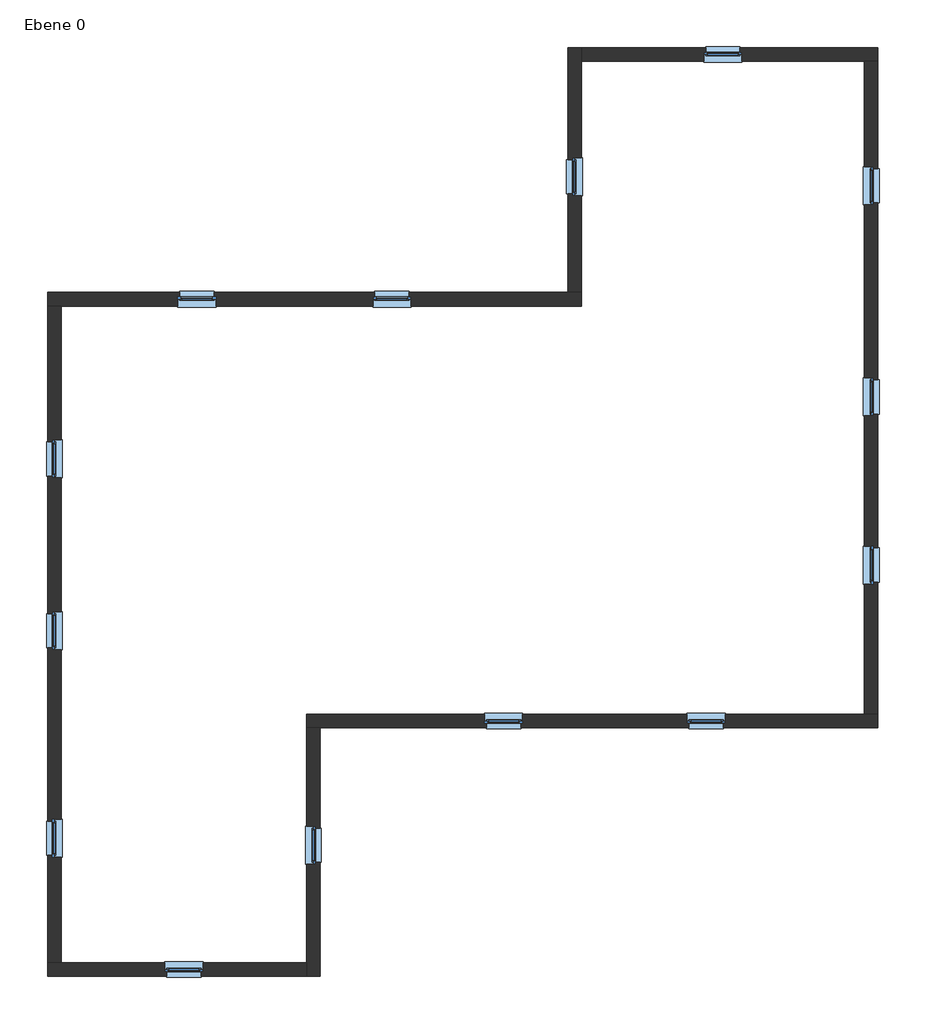
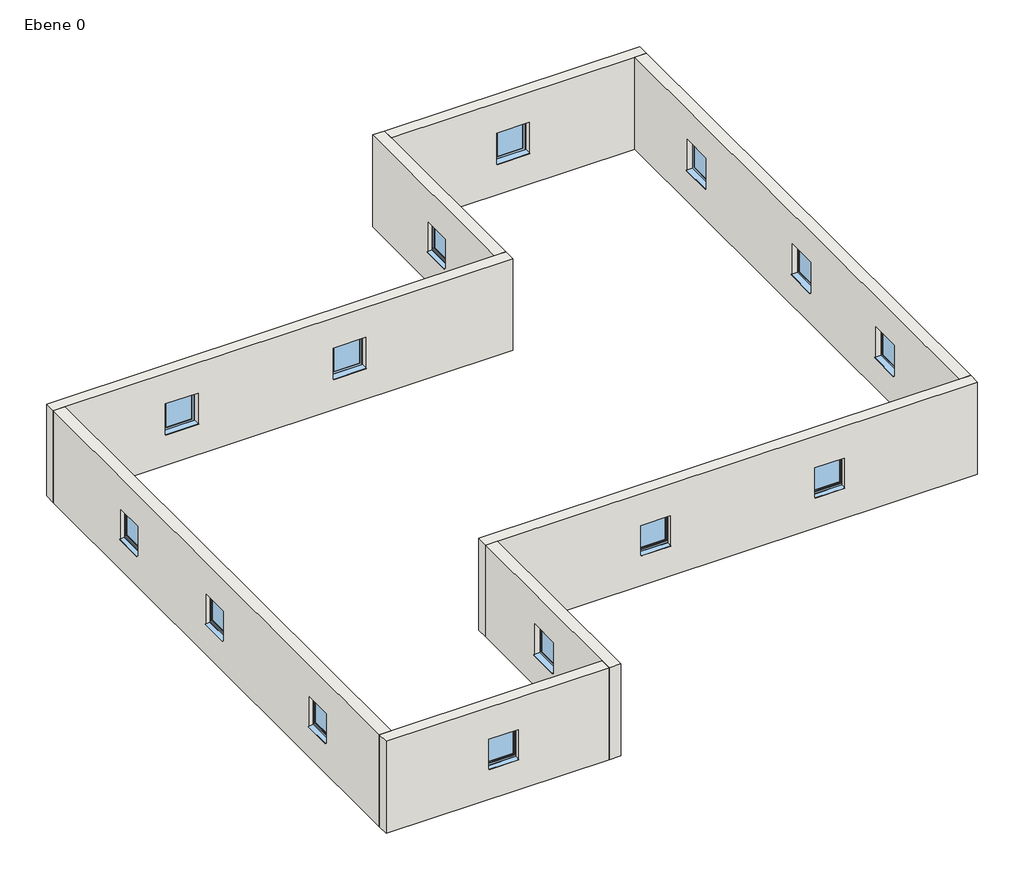
# One storey: 14 windows, 8 walls.
"""IFC4 building model written with IfcOpenShell, lengths in millimetres."""

import ifcopenshell
import ifcopenshell.guid

model = None  # the IFC model being written
_history = None  # IfcOwnerHistory: only IFC2X3 demands one
_inside = {}  # id of a spatial element -> (the spatial element, [elements in it])
_under = {}  # id of a project, library or spatial element -> (it, [spatial elements below it])
_declared = {}  # id of a project -> (the project, [libraries it declares])
_typed = {}  # id of a type object -> (the type object, [elements of that type])
_made_of = {}  # id of a material, layer set ... -> (it, [elements and type objects made of it])


def new_model(schema):
    """Start an empty IFC model of exactly this schema.

    Asked for "IFC4X3", IfcOpenShell would pick the latest addendum, in which some entities
    have other attributes; the version numbers below select the first issue.
    IFC2X3 requires an IfcOwnerHistory on every rooted entity: one is made here for all.
    """
    global model, _history
    if schema == "IFC4X3":
        model = ifcopenshell.file(schema_version=(4, 3, 0, 0))
    else:
        model = ifcopenshell.file(schema=schema)
    _inside.clear()
    _under.clear()
    _declared.clear()
    _typed.clear()
    _made_of.clear()
    _history = None
    if model.schema == "IFC2X3":
        org = make("IfcOrganization", Name="unknown")
        user = make(
            "IfcPersonAndOrganization",
            ThePerson=make("IfcPerson", FamilyName="unknown"),
            TheOrganization=org,
        )
        app = make(
            "IfcApplication",
            ApplicationDeveloper=org,
            Version="unknown",
            ApplicationFullName="unknown",
            ApplicationIdentifier="unknown",
        )
        _history = make(
            "IfcOwnerHistory",
            OwningUser=user,
            OwningApplication=app,
            ChangeAction="ADDED",
            CreationDate=0,
        )
    return model


def make(cls, **values):
    """One entity of the class cls with the attributes given. An attribute that is None is left unset."""
    return model.create_entity(
        cls, **{name: value for name, value in values.items() if value is not None}
    )


def rooted(cls, **values):
    """An entity with a GlobalId (a new one), such as an element, a storey or a relation."""
    return make(cls, GlobalId=ifcopenshell.guid.new(), OwnerHistory=_history, **values)


def si_unit(unit_type, name, prefix=None):
    """IfcSIUnit, for example si_unit("LENGTHUNIT", "METRE", prefix="MILLI")."""
    return make("IfcSIUnit", UnitType=unit_type, Prefix=prefix, Name=name)


def assignment(units):
    """IfcUnitAssignment: the units of a project."""
    return None if units is None else make("IfcUnitAssignment", Units=units)


def point(xyz):
    """IfcCartesianPoint."""
    return None if xyz is None else make("IfcCartesianPoint", Coordinates=xyz)


def direction(xyz):
    """IfcDirection."""
    return None if xyz is None else make("IfcDirection", DirectionRatios=xyz)


def frame(location, z_axis=None, x_axis=None):
    """IfcAxis2Placement3D, a coordinate frame: its origin and axes. An axis left out is left unset."""
    return make(
        "IfcAxis2Placement3D",
        Location=point(location),
        Axis=direction(z_axis),
        RefDirection=direction(x_axis),
    )


def origin():
    """The frame at (0, 0, 0) with its axes left unset."""
    return frame((0.0, 0.0, 0.0))


def place(relative_to, where):
    """IfcLocalPlacement: puts the frame where relative to a parent placement (None: the world)."""
    return make(
        "IfcLocalPlacement", PlacementRelTo=relative_to, RelativePlacement=where
    )


def context(
    kind, dimensions, precision=None, world=None, true_north=None, identifier=None
):
    """IfcGeometricRepresentationContext, for example the 3D "Model" context."""
    return make(
        "IfcGeometricRepresentationContext",
        ContextIdentifier=identifier,
        ContextType=kind,
        CoordinateSpaceDimension=dimensions,
        Precision=precision,
        WorldCoordinateSystem=world,
        TrueNorth=true_north,
    )


def project(units=None, contexts=None):
    """IfcProject with its units and contexts."""
    return rooted(
        "IfcProject",
        Name="project",
        RepresentationContexts=contexts,
        UnitsInContext=assignment(units),
    )


def spatial(cls, under=None, at=None, **own):
    """A site, building, storey or space (cls), placed at a placement, below another one or the project."""
    s = rooted(cls, ObjectPlacement=at, **own)
    if under is not None:
        _under.setdefault(under.id(), (under, []))[1].append(s)
    return s


def polyline(points):
    """IfcPolyline through the points."""
    return make("IfcPolyline", Points=[point(p) for p in points])


def outline(outer, holes=None, kind="AREA"):
    """IfcArbitraryClosedProfileDef: a profile drawn as a closed curve; with holes, ...WithVoids."""
    if holes is None:
        return make("IfcArbitraryClosedProfileDef", ProfileType=kind, OuterCurve=outer)
    return make(
        "IfcArbitraryProfileDefWithVoids",
        ProfileType=kind,
        OuterCurve=outer,
        InnerCurves=holes,
    )


def extrude(swept, where, along, depth):
    """IfcExtrudedAreaSolid: the profile swept, set in the frame where, extruded along a direction by depth."""
    return make(
        "IfcExtrudedAreaSolid",
        SweptArea=swept,
        Position=where,
        ExtrudedDirection=direction(along),
        Depth=depth,
    )


def faces_of(points, faces, orient=None, outer=None):
    """IfcFace entities. A face is a list of loops; a loop is a list of indices into points, from 0.

    orient and outer hold one flag for each loop. By default every Orientation is true, the
    first loop of a face is its IfcFaceOuterBound and the others are IfcFaceBound.
    """
    made = []
    for i, loops in enumerate(faces):
        bounds = []
        for j, loop in enumerate(loops):
            is_outer = j == 0 if outer is None else outer[i][j]
            bounds.append(
                make(
                    "IfcFaceOuterBound" if is_outer else "IfcFaceBound",
                    Bound=make("IfcPolyLoop", Polygon=[points[k] for k in loop]),
                    Orientation=True if orient is None else orient[i][j],
                )
            )
        made.append(make("IfcFace", Bounds=bounds))
    return made


def faceted_brep(points, faces, orient=None, outer=None, voids=None):
    """IfcFacetedBrep: a solid bounded by flat faces; with voids (closed shells), ...WithVoids."""
    shared = [point(p) for p in points]
    hull = make("IfcClosedShell", CfsFaces=faces_of(shared, faces, orient, outer))
    if voids is None:
        return make("IfcFacetedBrep", Outer=hull)
    return make(
        "IfcFacetedBrepWithVoids",
        Outer=hull,
        Voids=[
            make(cls, CfsFaces=faces_of(shared, fs, o, b)) for cls, fs, o, b in voids
        ],
    )


def shape(context_of_items, identifier, shape_type, items):
    """IfcShapeRepresentation: the items that make up one representation, for example the "Body"."""
    return make(
        "IfcShapeRepresentation",
        ContextOfItems=context_of_items,
        RepresentationIdentifier=identifier,
        RepresentationType=shape_type,
        Items=items,
    )


def source(mapping_origin, context_of_items, identifier, shape_type, items):
    """IfcRepresentationMap: a shape defined once, which mapped items show again and again."""
    return make(
        "IfcRepresentationMap",
        MappingOrigin=mapping_origin,
        MappedRepresentation=shape(context_of_items, identifier, shape_type, items),
    )


def transform(
    local_origin,
    x_axis=None,
    y_axis=None,
    z_axis=None,
    scale=None,
    scale2=None,
    scale3=None,
    uniform=True,
):
    """IfcCartesianTransformationOperator3D, or its non-uniform kind. x_axis, y_axis, z_axis: its Axis1, 2, 3."""
    if uniform:
        return make(
            "IfcCartesianTransformationOperator3D",
            Axis1=direction(x_axis),
            Axis2=direction(y_axis),
            LocalOrigin=point(local_origin),
            Scale=scale,
            Axis3=direction(z_axis),
        )
    return make(
        "IfcCartesianTransformationOperator3DnonUniform",
        Axis1=direction(x_axis),
        Axis2=direction(y_axis),
        LocalOrigin=point(local_origin),
        Scale=scale,
        Axis3=direction(z_axis),
        Scale2=scale2,
        Scale3=scale3,
    )


def mapped(mapping_source, mapping_target):
    """IfcMappedItem: shows the shape of a source again, moved by a transform."""
    return make(
        "IfcMappedItem", MappingSource=mapping_source, MappingTarget=mapping_target
    )


def made_of(thing, what):
    """Note that an element or type object is made of a material, layer set ...; save() writes the relation."""
    if what is not None:
        _made_of.setdefault(what.id(), (what, []))[1].append(thing)
    return thing


def element(
    cls,
    number,
    at=None,
    inside=None,
    cuts=None,
    type_object=None,
    material=None,
    context=None,
    identifier="Body",
    shape_type=None,
    held_by="IfcProductDefinitionShape",
    body=None,
    shapes=None,
    **own,
):
    """One element of the class cls, such as IfcWall. Its Tag is "e" and its number.

    at: its placement. inside: the storey or other place that contains it. cuts: it is an
    opening in that element (IfcRelVoidsElement). A single representation is given by context,
    identifier, shape_type and body (its items); several are given by shapes. held_by: the class
    of the entity that holds the representations. save() writes the other relations.
    """
    e = rooted(cls, Tag="e%d" % number, ObjectPlacement=at, **own)
    if body is not None:
        shapes = [shape(context, identifier, shape_type, body)]
    if shapes is not None:
        e.Representation = make(held_by, Representations=shapes)
    if inside is not None:
        _inside.setdefault(inside.id(), (inside, []))[1].append(e)
    if cuts is not None:
        rooted(
            "IfcRelVoidsElement", RelatingBuildingElement=cuts, RelatedOpeningElement=e
        )
    if type_object is not None:
        _typed.setdefault(type_object.id(), (type_object, []))[1].append(e)
    return made_of(e, material)


def aggregate(whole, parts):
    """IfcRelAggregates: a whole, such as a stair, and the parts it consists of."""
    return rooted("IfcRelAggregates", RelatingObject=whole, RelatedObjects=parts)


def save(model, path):
    """Write the relations noted so far, then the file.

    IfcRelAggregates (storeys below a building ...), IfcRelContainedInSpatialStructure (elements
    in a storey), IfcRelDefinesByType, IfcRelAssociatesMaterial and IfcRelDeclares: one each for
    every whole, place, type object, material and project.
    """
    for whole, parts in _under.values():
        aggregate(whole, parts)
    for where, things in _inside.values():
        rooted(
            "IfcRelContainedInSpatialStructure",
            RelatedElements=things,
            RelatingStructure=where,
        )
    for kind, things in _typed.values():
        rooted("IfcRelDefinesByType", RelatedObjects=things, RelatingType=kind)
    for what, things in _made_of.values():
        rooted("IfcRelAssociatesMaterial", RelatedObjects=things, RelatingMaterial=what)
    for by, libraries in _declared.values():
        rooted("IfcRelDeclares", RelatingContext=by, RelatedDefinitions=libraries)
    model.write(path)


def window_1_01_x_1_01_b7243dc8(model_context):
    return source(origin(), model_context, "Body", "SolidModel", [
        extrude(outline(polyline([(-525.0, -210.0), (-525.0, 0.0), (485.0, 0.0), (485.0, -210.0), (-525.0, -210.0)])), frame((0.0, 0.0, 1005.0), z_axis=(0.0, 0.0, 1.0), x_axis=(1.0, 0.0, 0.0)), (0.0, 0.0, 1.0), 15.0),
        extrude(outline(polyline([(375.0, -15.0), (-415.0, -15.0), (-415.0, 15.0), (375.0, 15.0), (375.0, -15.0)])), frame((0.0, 0.0, 1110.0), z_axis=(0.0, 0.0, 1.0), x_axis=(1.0, 0.0, 0.0)), (0.0, 0.0, 1.0), 790.0),
        extrude(outline(polyline([(70.0221543, 1020.0), (210.0, 1000.0), (210.0, 990.0), (208.0, 990.0), (208.0, 998.3604634), (69.8240723, 1018.0), (60.0, 1018.0), (60.0, 1020.0), (70.0221543, 1020.0)])), frame((-475.0, 0.0, 0.0), z_axis=(1.0, 0.0, 0.0), x_axis=(0.0, 1.0, 0.0)), (0.0, 0.0, 1.0), 910.0),
        extrude(outline(polyline([(2010.0, 485.0), (2010.0, -525.0), (1000.0, -525.0), (1000.0, 485.0), (2010.0, 485.0)]), holes=[polyline([(1930.0, 405.0), (1080.0, 405.0), (1080.0, -445.0), (1930.0, -445.0), (1930.0, 405.0)])]), frame((0.0, 0.0, 0.0), z_axis=(0.0, 1.0, 0.0), x_axis=(0.0, 0.0, 1.0)), (0.0, 0.0, 1.0), 60.0),
        faceted_brep([(435.0, 0.0, 1960.0), (435.0, -30.0, 1960.0), (435.0, -30.0, 1050.0), (435.0, 0.0, 1050.0), (-475.0, -30.0, 1960.0), (-475.0, -30.0, 1050.0), (375.0, -30.0, 1110.0), (-415.0, -30.0, 1110.0), (-415.0, -30.0, 1900.0), (375.0, -30.0, 1900.0), (-475.0, 0.0, 1050.0), (-475.0, 0.0, 1960.0), (405.0, 0.0, 1930.0), (-445.0, 0.0, 1930.0), (-445.0, 0.0, 1080.0), (405.0, 0.0, 1080.0), (405.0, 30.0, 1930.0), (405.0, 30.0, 1080.0), (-445.0, 30.0, 1080.0), (-445.0, 30.0, 1930.0), (375.0, 30.0, 1900.0), (-415.0, 30.0, 1900.0), (-415.0, 30.0, 1110.0), (375.0, 30.0, 1110.0)], [[[0, 1, 2, 3]], [[1, 4, 5, 2], [6, 7, 8, 9]], [[3, 2, 5, 10]], [[3, 10, 11, 0], [12, 13, 14, 15]], [[16, 12, 15, 17]], [[17, 15, 14, 18]], [[17, 18, 19, 16], [20, 21, 22, 23]], [[9, 20, 23, 6]], [[6, 23, 22, 7]], [[10, 5, 4, 11]], [[18, 14, 13, 19]], [[7, 22, 21, 8]], [[11, 4, 1, 0]], [[19, 13, 12, 16]], [[8, 21, 20, 9]]]),
    ])


model = new_model("IFC4")

# Units and contexts
model_context = context("Model", 3, world=origin())
ifc_project = project(units=[si_unit("LENGTHUNIT", "METRE", prefix="MILLI")], contexts=[model_context])

# Site, building, storey
site = spatial("IfcSite", under=ifc_project)
building = spatial("IfcBuilding", under=site)
storey = spatial("IfcBuildingStorey", under=building, Name="Ebene 0", Elevation=0.0)

# Walls
placement = place(None, origin())
element("IfcWall", 1, ObjectType="MW 24.0 WD 12.0", at=placement, inside=storey, context=model_context, shape_type="Brep", body=[
    faceted_brep([(-13369.6797169, 6985.6067473, 0.0), (-13009.6797169, 6985.6067473, 0.0), (810.3202831, 6985.6067473, 0.0), (810.3202831, 6985.6067473, 3000.0), (-13009.6797169, 6985.6067473, 3000.0), (-13369.6797169, 6985.6067473, 3000.0), (-8899.6797169, 6985.6067473, 1000.0), (-9909.6797169, 6985.6067473, 1000.0), (-9909.6797169, 6985.6067473, 2010.0), (-8899.6797169, 6985.6067473, 2010.0), (-3719.6797169, 6985.6067473, 1000.0), (-4729.6797169, 6985.6067473, 1000.0), (-4729.6797169, 6985.6067473, 2010.0), (-3719.6797169, 6985.6067473, 2010.0), (-13369.6797169, 7345.6067473, 0.0), (-13369.6797169, 7345.6067473, 3000.0), (450.3202831, 7345.6067473, 3000.0), (810.3202831, 7345.6067473, 3000.0), (810.3202831, 7345.6067473, 0.0), (450.3202831, 7345.6067473, 0.0), (-8949.6797169, 7345.6067473, 1960.0), (-9859.6797169, 7345.6067473, 1960.0), (-9859.6797169, 7345.6067473, 1000.0), (-8949.6797169, 7345.6067473, 1000.0), (-3769.6797169, 7345.6067473, 1960.0), (-4679.6797169, 7345.6067473, 1960.0), (-4679.6797169, 7345.6067473, 1000.0), (-3769.6797169, 7345.6067473, 1000.0), (-8949.6797169, 7225.6067473, 1960.0), (-9859.6797169, 7225.6067473, 1960.0), (-9859.6797169, 7225.6067473, 1000.0), (-8949.6797169, 7225.6067473, 1000.0), (-9909.6797169, 7225.6067473, 1000.0), (-8899.6797169, 7225.6067473, 1000.0), (-9909.6797169, 7225.6067473, 2010.0), (-8899.6797169, 7225.6067473, 2010.0), (-3769.6797169, 7225.6067473, 1960.0), (-4679.6797169, 7225.6067473, 1960.0), (-4679.6797169, 7225.6067473, 1000.0), (-3769.6797169, 7225.6067473, 1000.0), (-4729.6797169, 7225.6067473, 1000.0), (-3719.6797169, 7225.6067473, 1000.0), (-4729.6797169, 7225.6067473, 2010.0), (-3719.6797169, 7225.6067473, 2010.0)], [[[0, 1, 2, 3, 4, 5], [6, 7, 8, 9], [10, 11, 12, 13]], [[14, 15, 16, 17, 18, 19], [20, 21, 22, 23], [24, 25, 26, 27]], [[2, 1, 0, 14, 19, 18]], [[5, 4, 3, 17, 16, 15]], [[0, 5, 15, 14]], [[3, 2, 18, 17]], [[20, 28, 29, 21]], [[21, 29, 30, 22]], [[28, 20, 23, 31]], [[22, 30, 32, 7, 6, 33, 31, 23]], [[34, 35, 9, 8]], [[35, 33, 6, 9]], [[35, 34, 32, 30, 29, 28, 31, 33]], [[32, 34, 8, 7]], [[24, 36, 37, 25]], [[25, 37, 38, 26]], [[36, 24, 27, 39]], [[26, 38, 40, 11, 10, 41, 39, 27]], [[42, 43, 13, 12]], [[43, 41, 10, 13]], [[43, 42, 40, 38, 37, 36, 39, 41]], [[40, 42, 12, 11]]]),
])
element("IfcWall", 2, ObjectType="MW 24.0 WD 12.0", at=placement, inside=storey, context=model_context, shape_type="Brep", body=[
    faceted_brep([(-13009.6797169, -10454.3932527, 0.0), (-13009.6797169, 6985.6067473, 0.0), (-13009.6797169, 6985.6067473, 3000.0), (-13009.6797169, -10454.3932527, 3000.0), (-13009.6797169, -6644.3932527, 1000.0), (-13009.6797169, -7654.3932527, 1000.0), (-13009.6797169, -7654.3932527, 2010.0), (-13009.6797169, -6644.3932527, 2010.0), (-13009.6797169, -1134.3932527, 1000.0), (-13009.6797169, -2144.3932527, 1000.0), (-13009.6797169, -2144.3932527, 2010.0), (-13009.6797169, -1134.3932527, 2010.0), (-13009.6797169, 3430.6067473, 1000.0), (-13009.6797169, 2420.6067473, 1000.0), (-13009.6797169, 2420.6067473, 2010.0), (-13009.6797169, 3430.6067473, 2010.0), (-13369.6797169, -10454.3932527, 0.0), (-13369.6797169, -10454.3932527, 3000.0), (-13369.6797169, 6985.6067473, 3000.0), (-13369.6797169, 6985.6067473, 0.0), (-13369.6797169, -6694.3932527, 1960.0), (-13369.6797169, -7604.3932527, 1960.0), (-13369.6797169, -7604.3932527, 1000.0), (-13369.6797169, -6694.3932527, 1000.0), (-13369.6797169, -1184.3932527, 1960.0), (-13369.6797169, -2094.3932527, 1960.0), (-13369.6797169, -2094.3932527, 1000.0), (-13369.6797169, -1184.3932527, 1000.0), (-13369.6797169, 3380.6067473, 1960.0), (-13369.6797169, 2470.6067473, 1960.0), (-13369.6797169, 2470.6067473, 1000.0), (-13369.6797169, 3380.6067473, 1000.0), (-13249.6797169, -6694.3932527, 1960.0), (-13249.6797169, -7604.3932527, 1960.0), (-13249.6797169, -7604.3932527, 1000.0), (-13249.6797169, -6694.3932527, 1000.0), (-13249.6797169, -7654.3932527, 1000.0), (-13249.6797169, -6644.3932527, 1000.0), (-13249.6797169, -7654.3932527, 2010.0), (-13249.6797169, -6644.3932527, 2010.0), (-13249.6797169, -1184.3932527, 1960.0), (-13249.6797169, -2094.3932527, 1960.0), (-13249.6797169, -2094.3932527, 1000.0), (-13249.6797169, -1184.3932527, 1000.0), (-13249.6797169, -2144.3932527, 1000.0), (-13249.6797169, -1134.3932527, 1000.0), (-13249.6797169, -2144.3932527, 2010.0), (-13249.6797169, -1134.3932527, 2010.0), (-13249.6797169, 3380.6067473, 1960.0), (-13249.6797169, 2470.6067473, 1960.0), (-13249.6797169, 2470.6067473, 1000.0), (-13249.6797169, 3380.6067473, 1000.0), (-13249.6797169, 2420.6067473, 1000.0), (-13249.6797169, 3430.6067473, 1000.0), (-13249.6797169, 2420.6067473, 2010.0), (-13249.6797169, 3430.6067473, 2010.0)], [[[0, 1, 2, 3], [4, 5, 6, 7], [8, 9, 10, 11], [12, 13, 14, 15]], [[16, 17, 18, 19], [20, 21, 22, 23], [24, 25, 26, 27], [28, 29, 30, 31]], [[1, 0, 16, 19]], [[3, 2, 18, 17]], [[2, 1, 19, 18]], [[0, 3, 17, 16]], [[20, 32, 33, 21]], [[21, 33, 34, 22]], [[32, 20, 23, 35]], [[22, 34, 36, 5, 4, 37, 35, 23]], [[38, 39, 7, 6]], [[39, 37, 4, 7]], [[39, 38, 36, 34, 33, 32, 35, 37]], [[36, 38, 6, 5]], [[24, 40, 41, 25]], [[25, 41, 42, 26]], [[40, 24, 27, 43]], [[26, 42, 44, 9, 8, 45, 43, 27]], [[46, 47, 11, 10]], [[47, 45, 8, 11]], [[47, 46, 44, 42, 41, 40, 43, 45]], [[44, 46, 10, 9]], [[28, 48, 49, 29]], [[29, 49, 50, 30]], [[48, 28, 31, 51]], [[30, 50, 52, 13, 12, 53, 51, 31]], [[54, 55, 15, 14]], [[55, 53, 12, 15]], [[55, 54, 52, 50, 49, 48, 51, 53]], [[52, 54, 14, 13]]]),
])
element("IfcWall", 3, ObjectType="MW 24.0 WD 12.0", at=placement, inside=storey, context=model_context, shape_type="Brep", body=[
    faceted_brep([(8690.3202831, -3854.3932527, 0.0), (8330.3202831, -3854.3932527, 0.0), (-6489.6797169, -3854.3932527, 0.0), (-6489.6797169, -3854.3932527, 3000.0), (8330.3202831, -3854.3932527, 3000.0), (8690.3202831, -3854.3932527, 3000.0), (3620.3202831, -3854.3932527, 1000.0), (4630.3202831, -3854.3932527, 1000.0), (4630.3202831, -3854.3932527, 2010.0), (3620.3202831, -3854.3932527, 2010.0), (-1759.6797169, -3854.3932527, 1000.0), (-749.6797169, -3854.3932527, 1000.0), (-749.6797169, -3854.3932527, 2010.0), (-1759.6797169, -3854.3932527, 2010.0), (8690.3202831, -4214.3932527, 0.0), (8690.3202831, -4214.3932527, 3000.0), (-6129.6797169, -4214.3932527, 3000.0), (-6489.6797169, -4214.3932527, 3000.0), (-6489.6797169, -4214.3932527, 0.0), (-6129.6797169, -4214.3932527, 0.0), (3670.3202831, -4214.3932527, 1960.0), (4580.3202831, -4214.3932527, 1960.0), (4580.3202831, -4214.3932527, 1000.0), (3670.3202831, -4214.3932527, 1000.0), (-1709.6797169, -4214.3932527, 1960.0), (-799.6797169, -4214.3932527, 1960.0), (-799.6797169, -4214.3932527, 1000.0), (-1709.6797169, -4214.3932527, 1000.0), (3670.3202831, -4094.3932527, 1960.0), (4580.3202831, -4094.3932527, 1960.0), (4580.3202831, -4094.3932527, 1000.0), (3670.3202831, -4094.3932527, 1000.0), (4630.3202831, -4094.3932527, 1000.0), (3620.3202831, -4094.3932527, 1000.0), (4630.3202831, -4094.3932527, 2010.0), (3620.3202831, -4094.3932527, 2010.0), (-1709.6797169, -4094.3932527, 1960.0), (-799.6797169, -4094.3932527, 1960.0), (-799.6797169, -4094.3932527, 1000.0), (-1709.6797169, -4094.3932527, 1000.0), (-749.6797169, -4094.3932527, 1000.0), (-1759.6797169, -4094.3932527, 1000.0), (-749.6797169, -4094.3932527, 2010.0), (-1759.6797169, -4094.3932527, 2010.0)], [[[0, 1, 2, 3, 4, 5], [6, 7, 8, 9], [10, 11, 12, 13]], [[14, 15, 16, 17, 18, 19], [20, 21, 22, 23], [24, 25, 26, 27]], [[2, 1, 0, 14, 19, 18]], [[5, 4, 3, 17, 16, 15]], [[0, 5, 15, 14]], [[3, 2, 18, 17]], [[20, 28, 29, 21]], [[21, 29, 30, 22]], [[28, 20, 23, 31]], [[22, 30, 32, 7, 6, 33, 31, 23]], [[34, 35, 9, 8]], [[35, 33, 6, 9]], [[35, 34, 32, 30, 29, 28, 31, 33]], [[32, 34, 8, 7]], [[24, 36, 37, 25]], [[25, 37, 38, 26]], [[36, 24, 27, 39]], [[26, 38, 40, 11, 10, 41, 39, 27]], [[42, 43, 13, 12]], [[43, 41, 10, 13]], [[43, 42, 40, 38, 37, 36, 39, 41]], [[40, 42, 12, 11]]]),
])
element("IfcWall", 4, ObjectType="MW 24.0 WD 12.0", at=placement, inside=storey, context=model_context, shape_type="Brep", body=[
    faceted_brep([(8330.3202831, 13485.6067473, 0.0), (8330.3202831, -3854.3932527, 0.0), (8330.3202831, -3854.3932527, 3000.0), (8330.3202831, 13485.6067473, 3000.0), (8330.3202831, 9675.6067473, 1000.0), (8330.3202831, 10685.6067473, 1000.0), (8330.3202831, 10685.6067473, 2010.0), (8330.3202831, 9675.6067473, 2010.0), (8330.3202831, 4065.6067473, 1000.0), (8330.3202831, 5075.6067473, 1000.0), (8330.3202831, 5075.6067473, 2010.0), (8330.3202831, 4065.6067473, 2010.0), (8330.3202831, -399.3932527, 1000.0), (8330.3202831, 610.6067473, 1000.0), (8330.3202831, 610.6067473, 2010.0), (8330.3202831, -399.3932527, 2010.0), (8690.3202831, 13485.6067473, 0.0), (8690.3202831, 13485.6067473, 3000.0), (8690.3202831, -3854.3932527, 3000.0), (8690.3202831, -3854.3932527, 0.0), (8690.3202831, 9725.6067473, 1960.0), (8690.3202831, 10635.6067473, 1960.0), (8690.3202831, 10635.6067473, 1000.0), (8690.3202831, 9725.6067473, 1000.0), (8690.3202831, 4115.6067473, 1960.0), (8690.3202831, 5025.6067473, 1960.0), (8690.3202831, 5025.6067473, 1000.0), (8690.3202831, 4115.6067473, 1000.0), (8690.3202831, -349.3932527, 1960.0), (8690.3202831, 560.6067473, 1960.0), (8690.3202831, 560.6067473, 1000.0), (8690.3202831, -349.3932527, 1000.0), (8570.3202831, 9725.6067473, 1960.0), (8570.3202831, 10635.6067473, 1960.0), (8570.3202831, 10635.6067473, 1000.0), (8570.3202831, 9725.6067473, 1000.0), (8570.3202831, 10685.6067473, 1000.0), (8570.3202831, 9675.6067473, 1000.0), (8570.3202831, 10685.6067473, 2010.0), (8570.3202831, 9675.6067473, 2010.0), (8570.3202831, 4115.6067473, 1960.0), (8570.3202831, 5025.6067473, 1960.0), (8570.3202831, 5025.6067473, 1000.0), (8570.3202831, 4115.6067473, 1000.0), (8570.3202831, 5075.6067473, 1000.0), (8570.3202831, 4065.6067473, 1000.0), (8570.3202831, 5075.6067473, 2010.0), (8570.3202831, 4065.6067473, 2010.0), (8570.3202831, -349.3932527, 1960.0), (8570.3202831, 560.6067473, 1960.0), (8570.3202831, 560.6067473, 1000.0), (8570.3202831, -349.3932527, 1000.0), (8570.3202831, 610.6067473, 1000.0), (8570.3202831, -399.3932527, 1000.0), (8570.3202831, 610.6067473, 2010.0), (8570.3202831, -399.3932527, 2010.0)], [[[0, 1, 2, 3], [4, 5, 6, 7], [8, 9, 10, 11], [12, 13, 14, 15]], [[16, 17, 18, 19], [20, 21, 22, 23], [24, 25, 26, 27], [28, 29, 30, 31]], [[1, 0, 16, 19]], [[3, 2, 18, 17]], [[2, 1, 19, 18]], [[0, 3, 17, 16]], [[20, 32, 33, 21]], [[21, 33, 34, 22]], [[32, 20, 23, 35]], [[22, 34, 36, 5, 4, 37, 35, 23]], [[38, 39, 7, 6]], [[39, 37, 4, 7]], [[39, 38, 36, 34, 33, 32, 35, 37]], [[36, 38, 6, 5]], [[24, 40, 41, 25]], [[25, 41, 42, 26]], [[40, 24, 27, 43]], [[26, 42, 44, 9, 8, 45, 43, 27]], [[46, 47, 11, 10]], [[47, 45, 8, 11]], [[47, 46, 44, 42, 41, 40, 43, 45]], [[44, 46, 10, 9]], [[28, 48, 49, 29]], [[29, 49, 50, 30]], [[48, 28, 31, 51]], [[30, 50, 52, 13, 12, 53, 51, 31]], [[54, 55, 15, 14]], [[55, 53, 12, 15]], [[55, 54, 52, 50, 49, 48, 51, 53]], [[52, 54, 14, 13]]]),
])
element("IfcWall", 5, ObjectType="MW 24.0 WD 12.0", at=placement, inside=storey, context=model_context, shape_type="Brep", body=[
    faceted_brep([(810.3202831, 7345.6067473, 0.0), (810.3202831, 13485.6067473, 0.0), (810.3202831, 13845.6067473, 0.0), (810.3202831, 13845.6067473, 3000.0), (810.3202831, 13485.6067473, 3000.0), (810.3202831, 7345.6067473, 3000.0), (810.3202831, 10920.6067473, 1000.0), (810.3202831, 9910.6067473, 1000.0), (810.3202831, 9910.6067473, 2010.0), (810.3202831, 10920.6067473, 2010.0), (450.3202831, 7345.6067473, 0.0), (450.3202831, 7345.6067473, 3000.0), (450.3202831, 13845.6067473, 3000.0), (450.3202831, 13845.6067473, 0.0), (450.3202831, 10870.6067473, 1960.0), (450.3202831, 9960.6067473, 1960.0), (450.3202831, 9960.6067473, 1000.0), (450.3202831, 10870.6067473, 1000.0), (570.3202831, 10870.6067473, 1960.0), (570.3202831, 9960.6067473, 1960.0), (570.3202831, 9960.6067473, 1000.0), (570.3202831, 10870.6067473, 1000.0), (570.3202831, 9910.6067473, 1000.0), (570.3202831, 10920.6067473, 1000.0), (570.3202831, 9910.6067473, 2010.0), (570.3202831, 10920.6067473, 2010.0)], [[[0, 1, 2, 3, 4, 5], [6, 7, 8, 9]], [[10, 11, 12, 13], [14, 15, 16, 17]], [[2, 1, 0, 10, 13]], [[5, 4, 3, 12, 11]], [[3, 2, 13, 12]], [[0, 5, 11, 10]], [[14, 18, 19, 15]], [[15, 19, 20, 16]], [[18, 14, 17, 21]], [[16, 20, 22, 7, 6, 23, 21, 17]], [[24, 25, 9, 8]], [[25, 23, 6, 9]], [[25, 24, 22, 20, 19, 18, 21, 23]], [[22, 24, 8, 7]]]),
])
element("IfcWall", 6, ObjectType="MW 24.0 WD 12.0", at=placement, inside=storey, context=model_context, shape_type="Brep", body=[
    faceted_brep([(810.3202831, 13485.6067473, 0.0), (8330.3202831, 13485.6067473, 0.0), (8690.3202831, 13485.6067473, 0.0), (8690.3202831, 13485.6067473, 3000.0), (8330.3202831, 13485.6067473, 3000.0), (810.3202831, 13485.6067473, 3000.0), (5075.3202831, 13485.6067473, 1000.0), (4065.3202831, 13485.6067473, 1000.0), (4065.3202831, 13485.6067473, 2010.0), (5075.3202831, 13485.6067473, 2010.0), (810.3202831, 13845.6067473, 0.0), (810.3202831, 13845.6067473, 3000.0), (8690.3202831, 13845.6067473, 3000.0), (8690.3202831, 13845.6067473, 0.0), (5025.3202831, 13845.6067473, 1960.0), (4115.3202831, 13845.6067473, 1960.0), (4115.3202831, 13845.6067473, 1000.0), (5025.3202831, 13845.6067473, 1000.0), (5025.3202831, 13725.6067473, 1960.0), (4115.3202831, 13725.6067473, 1960.0), (4115.3202831, 13725.6067473, 1000.0), (5025.3202831, 13725.6067473, 1000.0), (4065.3202831, 13725.6067473, 1000.0), (5075.3202831, 13725.6067473, 1000.0), (4065.3202831, 13725.6067473, 2010.0), (5075.3202831, 13725.6067473, 2010.0)], [[[0, 1, 2, 3, 4, 5], [6, 7, 8, 9]], [[10, 11, 12, 13], [14, 15, 16, 17]], [[2, 1, 0, 10, 13]], [[5, 4, 3, 12, 11]], [[0, 5, 11, 10]], [[3, 2, 13, 12]], [[14, 18, 19, 15]], [[15, 19, 20, 16]], [[18, 14, 17, 21]], [[16, 20, 22, 7, 6, 23, 21, 17]], [[24, 25, 9, 8]], [[25, 23, 6, 9]], [[25, 24, 22, 20, 19, 18, 21, 23]], [[22, 24, 8, 7]]]),
])
element("IfcWall", 7, ObjectType="MW 24.0 WD 12.0", at=placement, inside=storey, context=model_context, shape_type="Brep", body=[
    faceted_brep([(-6489.6797169, -4214.3932527, 0.0), (-6489.6797169, -10454.3932527, 0.0), (-6489.6797169, -10814.3932527, 0.0), (-6489.6797169, -10814.3932527, 3000.0), (-6489.6797169, -10454.3932527, 3000.0), (-6489.6797169, -4214.3932527, 3000.0), (-6489.6797169, -7839.3932527, 1000.0), (-6489.6797169, -6829.3932527, 1000.0), (-6489.6797169, -6829.3932527, 2010.0), (-6489.6797169, -7839.3932527, 2010.0), (-6129.6797169, -4214.3932527, 0.0), (-6129.6797169, -4214.3932527, 3000.0), (-6129.6797169, -10814.3932527, 3000.0), (-6129.6797169, -10814.3932527, 0.0), (-6129.6797169, -7789.3932527, 1960.0), (-6129.6797169, -6879.3932527, 1960.0), (-6129.6797169, -6879.3932527, 1000.0), (-6129.6797169, -7789.3932527, 1000.0), (-6249.6797169, -7789.3932527, 1960.0), (-6249.6797169, -6879.3932527, 1960.0), (-6249.6797169, -6879.3932527, 1000.0), (-6249.6797169, -7789.3932527, 1000.0), (-6249.6797169, -6829.3932527, 1000.0), (-6249.6797169, -7839.3932527, 1000.0), (-6249.6797169, -6829.3932527, 2010.0), (-6249.6797169, -7839.3932527, 2010.0)], [[[0, 1, 2, 3, 4, 5], [6, 7, 8, 9]], [[10, 11, 12, 13], [14, 15, 16, 17]], [[2, 1, 0, 10, 13]], [[5, 4, 3, 12, 11]], [[3, 2, 13, 12]], [[0, 5, 11, 10]], [[14, 18, 19, 15]], [[15, 19, 20, 16]], [[18, 14, 17, 21]], [[16, 20, 22, 7, 6, 23, 21, 17]], [[24, 25, 9, 8]], [[25, 23, 6, 9]], [[25, 24, 22, 20, 19, 18, 21, 23]], [[22, 24, 8, 7]]]),
])
element("IfcWall", 8, ObjectType="MW 24.0 WD 12.0", at=placement, inside=storey, context=model_context, shape_type="Brep", body=[
    faceted_brep([(-6489.6797169, -10454.3932527, 0.0), (-13009.6797169, -10454.3932527, 0.0), (-13369.6797169, -10454.3932527, 0.0), (-13369.6797169, -10454.3932527, 3000.0), (-13009.6797169, -10454.3932527, 3000.0), (-6489.6797169, -10454.3932527, 3000.0), (-10254.6797169, -10454.3932527, 1000.0), (-9244.6797169, -10454.3932527, 1000.0), (-9244.6797169, -10454.3932527, 2010.0), (-10254.6797169, -10454.3932527, 2010.0), (-6489.6797169, -10814.3932527, 0.0), (-6489.6797169, -10814.3932527, 3000.0), (-13369.6797169, -10814.3932527, 3000.0), (-13369.6797169, -10814.3932527, 0.0), (-10204.6797169, -10814.3932527, 1960.0), (-9294.6797169, -10814.3932527, 1960.0), (-9294.6797169, -10814.3932527, 1000.0), (-10204.6797169, -10814.3932527, 1000.0), (-10204.6797169, -10694.3932527, 1960.0), (-9294.6797169, -10694.3932527, 1960.0), (-9294.6797169, -10694.3932527, 1000.0), (-10204.6797169, -10694.3932527, 1000.0), (-9244.6797169, -10694.3932527, 1000.0), (-10254.6797169, -10694.3932527, 1000.0), (-9244.6797169, -10694.3932527, 2010.0), (-10254.6797169, -10694.3932527, 2010.0)], [[[0, 1, 2, 3, 4, 5], [6, 7, 8, 9]], [[10, 11, 12, 13], [14, 15, 16, 17]], [[2, 1, 0, 10, 13]], [[5, 4, 3, 12, 11]], [[0, 5, 11, 10]], [[3, 2, 13, 12]], [[14, 18, 19, 15]], [[15, 19, 20, 16]], [[18, 14, 17, 21]], [[16, 20, 22, 7, 6, 23, 21, 17]], [[24, 25, 9, 8]], [[25, 23, 6, 9]], [[25, 24, 22, 20, 19, 18, 21, 23]], [[22, 24, 8, 7]]]),
])

# Windows
window_1_01_x_1_01_shape = window_1_01_x_1_01_b7243dc8(model_context)
element("IfcWindow", 9, ObjectType="Fenster 1-flg - Anschlag : 1.01 x 1.01", at=placement, inside=storey, context=model_context, shape_type="MappedRepresentation", body=[
    mapped(window_1_01_x_1_01_shape, transform((-9384.6797169, 7165.6067473, 0.0), x_axis=(1.0, 0.0, 0.0), y_axis=(0.0, 1.0, 0.0), z_axis=(0.0, 0.0, 1.0))),
])
element("IfcWindow", 10, ObjectType="Fenster 1-flg - Anschlag : 1.01 x 1.01", at=placement, inside=storey, context=model_context, shape_type="MappedRepresentation", body=[
    mapped(window_1_01_x_1_01_shape, transform((-4204.6797169, 7165.6067473, 0.0), x_axis=(1.0, 0.0, 0.0), y_axis=(0.0, 1.0, 0.0), z_axis=(0.0, 0.0, 1.0))),
])
element("IfcWindow", 11, ObjectType="Fenster 1-flg - Anschlag : 1.01 x 1.01", at=placement, inside=storey, context=model_context, shape_type="MappedRepresentation", body=[
    mapped(window_1_01_x_1_01_shape, transform((4590.3202831, 13665.6067473, 0.0), x_axis=(1.0, 0.0, 0.0), y_axis=(0.0, 1.0, 0.0), z_axis=(0.0, 0.0, 1.0))),
])
element("IfcWindow", 12, ObjectType="Fenster 1-flg - Anschlag : 1.01 x 1.01", at=placement, inside=storey, context=model_context, shape_type="MappedRepresentation", body=[
    mapped(window_1_01_x_1_01_shape, transform((4105.3202831, -4034.3932527, 0.0), x_axis=(-1.0, 0.0, 0.0), y_axis=(0.0, -1.0, 0.0), z_axis=(0.0, 0.0, 1.0))),
])
element("IfcWindow", 13, ObjectType="Fenster 1-flg - Anschlag : 1.01 x 1.01", at=placement, inside=storey, context=model_context, shape_type="MappedRepresentation", body=[
    mapped(window_1_01_x_1_01_shape, transform((-1274.6797169, -4034.3932527, 0.0), x_axis=(-1.0, 0.0, 0.0), y_axis=(0.0, -1.0, 0.0), z_axis=(0.0, 0.0, 1.0))),
])
element("IfcWindow", 14, ObjectType="Fenster 1-flg - Anschlag : 1.01 x 1.01", at=placement, inside=storey, context=model_context, shape_type="MappedRepresentation", body=[
    mapped(window_1_01_x_1_01_shape, transform((-9769.6797169, -10634.3932527, 0.0), x_axis=(-1.0, 0.0, 0.0), y_axis=(0.0, -1.0, 0.0), z_axis=(0.0, 0.0, 1.0))),
])
element("IfcWindow", 15, ObjectType="Fenster 1-flg - Anschlag : 1.01 x 1.01", at=placement, inside=storey, context=model_context, shape_type="MappedRepresentation", body=[
    mapped(window_1_01_x_1_01_shape, transform((-6309.6797169, -7354.3932527, 0.0), x_axis=(0.0, -1.0, 0.0), y_axis=(1.0, 0.0, 0.0), z_axis=(0.0, 0.0, 1.0))),
])
element("IfcWindow", 16, ObjectType="Fenster 1-flg - Anschlag : 1.01 x 1.01", at=placement, inside=storey, context=model_context, shape_type="MappedRepresentation", body=[
    mapped(window_1_01_x_1_01_shape, transform((-13189.6797169, -7129.3932527, 0.0), x_axis=(0.0, 1.0, 0.0), y_axis=(-1.0, 0.0, 0.0), z_axis=(0.0, 0.0, 1.0))),
])
element("IfcWindow", 17, ObjectType="Fenster 1-flg - Anschlag : 1.01 x 1.01", at=placement, inside=storey, context=model_context, shape_type="MappedRepresentation", body=[
    mapped(window_1_01_x_1_01_shape, transform((-13189.6797169, -1619.3932527, 0.0), x_axis=(0.0, 1.0, 0.0), y_axis=(-1.0, 0.0, 0.0), z_axis=(0.0, 0.0, 1.0))),
])
element("IfcWindow", 18, ObjectType="Fenster 1-flg - Anschlag : 1.01 x 1.01", at=placement, inside=storey, context=model_context, shape_type="MappedRepresentation", body=[
    mapped(window_1_01_x_1_01_shape, transform((-13189.6797169, 2945.6067473, 0.0), x_axis=(0.0, 1.0, 0.0), y_axis=(-1.0, 0.0, 0.0), z_axis=(0.0, 0.0, 1.0))),
])
element("IfcWindow", 19, ObjectType="Fenster 1-flg - Anschlag : 1.01 x 1.01", at=placement, inside=storey, context=model_context, shape_type="MappedRepresentation", body=[
    mapped(window_1_01_x_1_01_shape, transform((630.3202831, 10435.6067473, 0.0), x_axis=(0.0, 1.0, 0.0), y_axis=(-1.0, 0.0, 0.0), z_axis=(0.0, 0.0, 1.0))),
])
element("IfcWindow", 20, ObjectType="Fenster 1-flg - Anschlag : 1.01 x 1.01", at=placement, inside=storey, context=model_context, shape_type="MappedRepresentation", body=[
    mapped(window_1_01_x_1_01_shape, transform((8510.3202831, 10160.6067473, 0.0), x_axis=(0.0, -1.0, 0.0), y_axis=(1.0, 0.0, 0.0), z_axis=(0.0, 0.0, 1.0))),
])
element("IfcWindow", 21, ObjectType="Fenster 1-flg - Anschlag : 1.01 x 1.01", at=placement, inside=storey, context=model_context, shape_type="MappedRepresentation", body=[
    mapped(window_1_01_x_1_01_shape, transform((8510.3202831, 4550.6067473, 0.0), x_axis=(0.0, -1.0, 0.0), y_axis=(1.0, 0.0, 0.0), z_axis=(0.0, 0.0, 1.0))),
])
element("IfcWindow", 22, ObjectType="Fenster 1-flg - Anschlag : 1.01 x 1.01", at=placement, inside=storey, context=model_context, shape_type="MappedRepresentation", body=[
    mapped(window_1_01_x_1_01_shape, transform((8510.3202831, 85.6067473, 0.0), x_axis=(0.0, -1.0, 0.0), y_axis=(1.0, 0.0, 0.0), z_axis=(0.0, 0.0, 1.0))),
])

save(model, "model.ifc")

# Revit data of these elements
# Project information
#   Projektausgabedatum = "Projekt Datum"
#   Projektstatus = "Projektstatus"
#   Kundenname = "Bauherr"
#   Projektadresse = "Projektadresse"
#   Projektname = "Projektname"
#   Projektnummer = "Projektnummer"
#   Verfasser Firma 1 = "Firma 1"
#   Verfasser Firma 2 = "Firma 2"
#   Verfasser PLZ Ort = "PLZ Ort"
#   Verfasser Strasse = "Strasse"
#   Verfasser Telefon = "Telefon"
#   Verfasser Telefax = "Telefax"
#   Verfasser eMail = "E-Mail"
# Type "MW 24.0 WD 12.0"
#   Type Comments = "Mehrschaliges Mauerwerk"
#   Description = "Mauerwerk 24.0 cm, Wärmedämmung 12.0 cm"
#   Width = 0.360 m
#   Layers, outside or top first: 0.120 m "Wärmedämmung - Hart" (function 3); 0.240 m "Mauerwerk - Ziegel, verputzt" (function 1)
# Type "Fenster 1-flg - Anschlag : 1.01 x 1.01"
#   Type Mark = "47"
#   Operation = "SinglePanel"
#   Keynote = "16.05.01"
#   Construction Type Id = "GSP4R"
#   Analytic Construction = "1/8 Zoll Pilkington-Verglasung einfach"
#   Visual Light Transmittance = 0.9
#   Thermal Resistance (R) = 0.1491 (m²·K)/W
#   Solar Heat Gain Coefficient = 0.86
#   Anschlagsbreite seitlich = 0.050 m
#   Rough Width = 1.010 m
#   Rough Height = 1.010 m
#   Heat Transfer Coefficient (U) = 6.7069 W/(m²·K)
#   Rahmentiefe = 0.060 m
#   Rahmenhöhe unten = 0.080 m
#   Rahmenhöhe oben = 0.080 m
#   Rahmenbreite = 0.080 m
#   Height = 1.010 m
#   Flügeltiefe = 0.060 m
#   Flügelbreite = 0.060 m
#   Einbautiefe (von außen) [instance default] = 0.120 m
#   Width = 1.010 m
#   Anschlagsbreite oben = 0.050 m
#   Klappflügel [instance default] = no
#   Öffnungsrichtung oben [instance default] = yes
#   Öffnungsrichtung in Draufsicht anzeigen [instance default] = no
#   Drehflügel [instance default] = yes
#   Rahmen [instance default] = none
#   Glas [instance default] = none
#   Flügel [instance default] = none
#   Fensterbank innen [instance default] = none
#   Fensterbank außen [instance default] = none
#   Wall Closure = (empty or 0)
# Elements 1, 2, 3, 4 (IfcWall, "MW 24.0 WD 12.0")
#   Top Offset = 0.000 m
#   Base Offset = 0.000 m
#   wall height = 3.000 m
#   Phase Created = Phase 1
#   Base Constraint = Ebene 0
#   Top Constraint = Ebene 1
#   Materials on its faces: "Standard - Wand", "Mauerwerk - Ziegel, verputzt", "Wärmedämmung - Hart"
# Elements 5, 6, 7, 8 (IfcWall, "MW 24.0 WD 12.0")
#   Top Offset = 0.000 m
#   Base Offset = 0.000 m
#   wall height = 3.000 m
#   Phase Created = Phase 1
#   Base Constraint = Ebene 0
#   Top Constraint = Ebene 1
#   Materials on its faces: "Standard - Wand", "Wärmedämmung - Hart", "Mauerwerk - Ziegel, verputzt"
# Element 9 (IfcWindow, "Fenster 1-flg - Anschlag : 1.01 x 1.01")
#   Mark = "1"
#   Einbautiefe (von außen) = 0.120 m
#   Öffnungsrichtung oben = yes
#   Öffnungsrichtung in Draufsicht anzeigen = no
#   Klappflügel = no
#   Drehflügel = yes
#   Rahmen = none
#   Glas = none
#   Flügel = none
#   Fensterbank innen = none
#   Fensterbank außen = none
#   Phase Created = Phase 1
#   Materials on its faces: "Kunststoff - Weiß", "Holz - Birke", "Glas"
# Element 10 (IfcWindow, "Fenster 1-flg - Anschlag : 1.01 x 1.01")
#   Mark = "2"
#   Einbautiefe (von außen) = 0.120 m
#   Öffnungsrichtung oben = yes
#   Öffnungsrichtung in Draufsicht anzeigen = no
#   Klappflügel = no
#   Drehflügel = yes
#   Rahmen = none
#   Glas = none
#   Flügel = none
#   Fensterbank innen = none
#   Fensterbank außen = none
#   Phase Created = Phase 1
#   Materials on its faces: "Kunststoff - Weiß", "Holz - Birke", "Glas"
# Element 11 (IfcWindow, "Fenster 1-flg - Anschlag : 1.01 x 1.01")
#   Mark = "3"
#   Einbautiefe (von außen) = 0.120 m
#   Öffnungsrichtung oben = yes
#   Öffnungsrichtung in Draufsicht anzeigen = no
#   Klappflügel = no
#   Drehflügel = yes
#   Rahmen = none
#   Glas = none
#   Flügel = none
#   Fensterbank innen = none
#   Fensterbank außen = none
#   Phase Created = Phase 1
#   Materials on its faces: "Kunststoff - Weiß", "Holz - Birke", "Glas"
# Element 12 (IfcWindow, "Fenster 1-flg - Anschlag : 1.01 x 1.01")
#   Mark = "4"
#   Einbautiefe (von außen) = 0.120 m
#   Öffnungsrichtung oben = yes
#   Öffnungsrichtung in Draufsicht anzeigen = no
#   Klappflügel = no
#   Drehflügel = yes
#   Rahmen = none
#   Glas = none
#   Flügel = none
#   Fensterbank innen = none
#   Fensterbank außen = none
#   Phase Created = Phase 1
#   Materials on its faces: "Kunststoff - Weiß", "Holz - Birke", "Glas"
# Element 13 (IfcWindow, "Fenster 1-flg - Anschlag : 1.01 x 1.01")
#   Mark = "5"
#   Einbautiefe (von außen) = 0.120 m
#   Öffnungsrichtung oben = yes
#   Öffnungsrichtung in Draufsicht anzeigen = no
#   Klappflügel = no
#   Drehflügel = yes
#   Rahmen = none
#   Glas = none
#   Flügel = none
#   Fensterbank innen = none
#   Fensterbank außen = none
#   Phase Created = Phase 1
#   Materials on its faces: "Kunststoff - Weiß", "Holz - Birke", "Glas"
# Element 14 (IfcWindow, "Fenster 1-flg - Anschlag : 1.01 x 1.01")
#   Mark = "6"
#   Einbautiefe (von außen) = 0.120 m
#   Öffnungsrichtung oben = yes
#   Öffnungsrichtung in Draufsicht anzeigen = no
#   Klappflügel = no
#   Drehflügel = yes
#   Rahmen = none
#   Glas = none
#   Flügel = none
#   Fensterbank innen = none
#   Fensterbank außen = none
#   Phase Created = Phase 1
#   Materials on its faces: "Kunststoff - Weiß", "Holz - Birke", "Glas"
# Element 15 (IfcWindow, "Fenster 1-flg - Anschlag : 1.01 x 1.01")
#   Mark = "7"
#   Einbautiefe (von außen) = 0.120 m
#   Öffnungsrichtung oben = yes
#   Öffnungsrichtung in Draufsicht anzeigen = no
#   Klappflügel = no
#   Drehflügel = yes
#   Rahmen = none
#   Glas = none
#   Flügel = none
#   Fensterbank innen = none
#   Fensterbank außen = none
#   Phase Created = Phase 1
#   Materials on its faces: "Kunststoff - Weiß", "Holz - Birke", "Glas"
# Element 16 (IfcWindow, "Fenster 1-flg - Anschlag : 1.01 x 1.01")
#   Mark = "8"
#   Einbautiefe (von außen) = 0.120 m
#   Öffnungsrichtung oben = yes
#   Öffnungsrichtung in Draufsicht anzeigen = no
#   Klappflügel = no
#   Drehflügel = yes
#   Rahmen = none
#   Glas = none
#   Flügel = none
#   Fensterbank innen = none
#   Fensterbank außen = none
#   Phase Created = Phase 1
#   Materials on its faces: "Kunststoff - Weiß", "Holz - Birke", "Glas"
# Element 17 (IfcWindow, "Fenster 1-flg - Anschlag : 1.01 x 1.01")
#   Mark = "9"
#   Einbautiefe (von außen) = 0.120 m
#   Öffnungsrichtung oben = yes
#   Öffnungsrichtung in Draufsicht anzeigen = no
#   Klappflügel = no
#   Drehflügel = yes
#   Rahmen = none
#   Glas = none
#   Flügel = none
#   Fensterbank innen = none
#   Fensterbank außen = none
#   Phase Created = Phase 1
#   Materials on its faces: "Kunststoff - Weiß", "Holz - Birke", "Glas"
# Element 18 (IfcWindow, "Fenster 1-flg - Anschlag : 1.01 x 1.01")
#   Mark = "10"
#   Einbautiefe (von außen) = 0.120 m
#   Öffnungsrichtung oben = yes
#   Öffnungsrichtung in Draufsicht anzeigen = no
#   Klappflügel = no
#   Drehflügel = yes
#   Rahmen = none
#   Glas = none
#   Flügel = none
#   Fensterbank innen = none
#   Fensterbank außen = none
#   Phase Created = Phase 1
#   Materials on its faces: "Kunststoff - Weiß", "Holz - Birke", "Glas"
# Element 19 (IfcWindow, "Fenster 1-flg - Anschlag : 1.01 x 1.01")
#   Mark = "11"
#   Einbautiefe (von außen) = 0.120 m
#   Öffnungsrichtung oben = yes
#   Öffnungsrichtung in Draufsicht anzeigen = no
#   Klappflügel = no
#   Drehflügel = yes
#   Rahmen = none
#   Glas = none
#   Flügel = none
#   Fensterbank innen = none
#   Fensterbank außen = none
#   Phase Created = Phase 1
#   Materials on its faces: "Kunststoff - Weiß", "Holz - Birke", "Glas"
# Element 20 (IfcWindow, "Fenster 1-flg - Anschlag : 1.01 x 1.01")
#   Mark = "12"
#   Einbautiefe (von außen) = 0.120 m
#   Öffnungsrichtung oben = yes
#   Öffnungsrichtung in Draufsicht anzeigen = no
#   Klappflügel = no
#   Drehflügel = yes
#   Rahmen = none
#   Glas = none
#   Flügel = none
#   Fensterbank innen = none
#   Fensterbank außen = none
#   Phase Created = Phase 1
#   Materials on its faces: "Kunststoff - Weiß", "Holz - Birke", "Glas"
# Element 21 (IfcWindow, "Fenster 1-flg - Anschlag : 1.01 x 1.01")
#   Mark = "13"
#   Einbautiefe (von außen) = 0.120 m
#   Öffnungsrichtung oben = yes
#   Öffnungsrichtung in Draufsicht anzeigen = no
#   Klappflügel = no
#   Drehflügel = yes
#   Rahmen = none
#   Glas = none
#   Flügel = none
#   Fensterbank innen = none
#   Fensterbank außen = none
#   Phase Created = Phase 1
#   Materials on its faces: "Kunststoff - Weiß", "Holz - Birke", "Glas"
# Element 22 (IfcWindow, "Fenster 1-flg - Anschlag : 1.01 x 1.01")
#   Mark = "14"
#   Einbautiefe (von außen) = 0.120 m
#   Öffnungsrichtung oben = yes
#   Öffnungsrichtung in Draufsicht anzeigen = no
#   Klappflügel = no
#   Drehflügel = yes
#   Rahmen = none
#   Glas = none
#   Flügel = none
#   Fensterbank innen = none
#   Fensterbank außen = none
#   Phase Created = Phase 1
#   Materials on its faces: "Kunststoff - Weiß", "Holz - Birke", "Glas"
# Materials
#   "Wärmedämmung - Hart": class "Putz", colour RGB 255 255 255, transparency 0, Description = "Äußere Oberfläche"
#   "Mauerwerk - Ziegel, verputzt": class "Putz", colour RGB 247 247 247, transparency 0, Cost = 0
#   "Standard - Wand": class "Putz", colour RGB 128 128 128, transparency 0, Description = "Äußere Oberfläche"
#   "Kunststoff - Weiß": class "Kunststoff", colour RGB 249 249 249, transparency 0
#   "Holz - Birke": class "Holz", colour RGB 213 164 103, transparency 0
#   "Glas": class "Glas", colour RGB 0 0 255, transparency 0.75, Comments = "Renderdarstellung nicht aktualisiert ", Cost = 0
